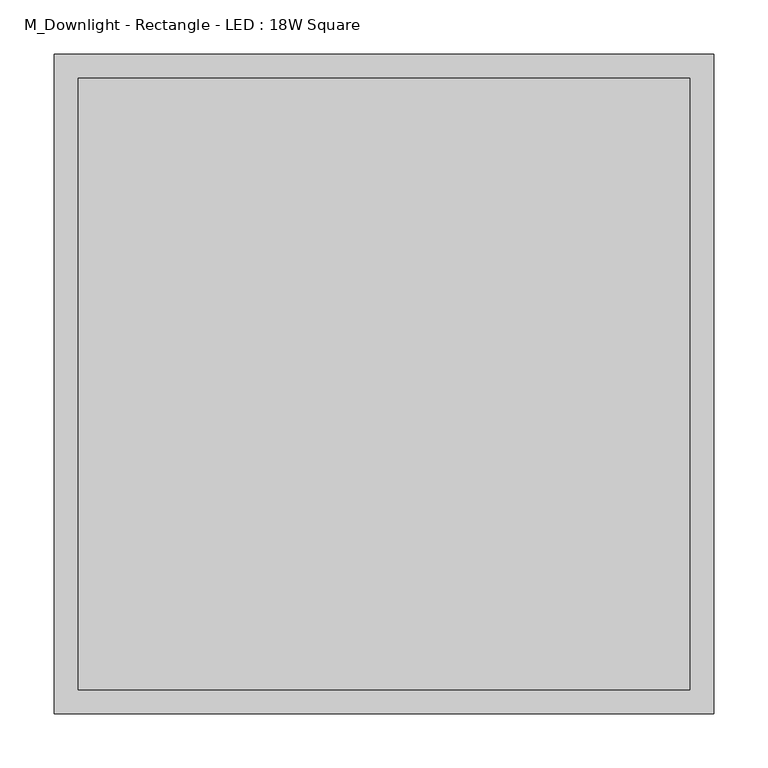
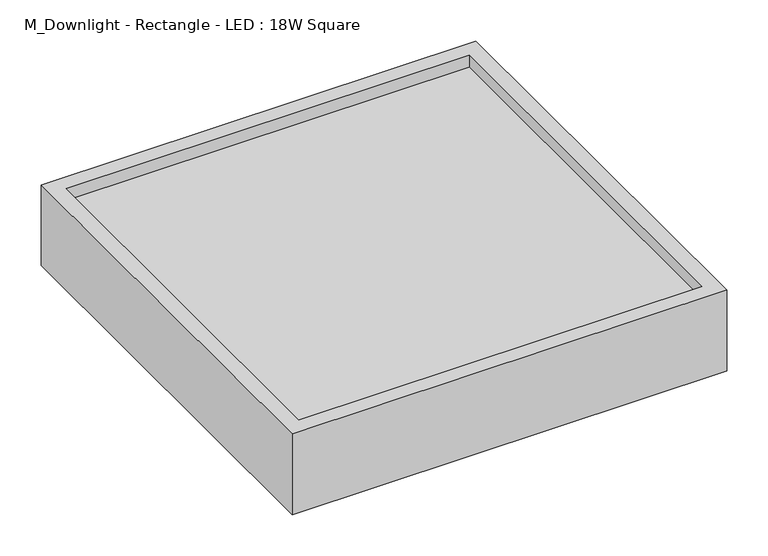
"""IFC4 building model written with IfcOpenShell, lengths in millimetres: light fixture geometry, M_Downlight - Rectangle - LED : 18W Square."""

from ifc_helpers import new_model, si_unit, frame, origin, place, context, project, spatial, polyline, outline, extrude, faceted_brep, source, transform, mapped, element, save


def m_downlight_rectangle_led_18w_square_4974df87(model_context):
    return source(origin(), model_context, "Body", "SolidModel", [
        extrude(outline(polyline([(282.775, 282.775), (282.775, -282.775), (-282.775, -282.775), (-282.775, 282.775), (282.775, 282.775)])), frame((0.0, 0.0, 84.7359902), z_axis=(0.0, 0.0, 1.0), x_axis=(1.0, 0.0, 0.0)), (0.0, 0.0, 1.0), 17.6320049),
        faceted_brep([(305.0, 305.0, 120.0), (-305.0, 305.0, 120.0), (-305.0, -305.0, 120.0), (305.0, -305.0, 120.0), (-282.775, 282.775, 120.0), (282.775, 282.775, 120.0), (282.775, -282.775, 120.0), (-282.775, -282.775, 120.0), (305.0, 305.0, 0.0), (305.0, -305.0, 0.0), (-305.0, -305.0, 0.0), (-305.0, 305.0, 0.0), (282.775, 282.775, 17.0719804), (-282.775, 282.775, 17.0719804), (-282.775, -282.775, 17.0719804), (282.775, -282.775, 17.0719804)], [[[0, 1, 2, 3], [4, 5, 6, 7]], [[8, 9, 10, 11]], [[1, 0, 8, 11]], [[2, 1, 11, 10]], [[3, 2, 10, 9]], [[0, 3, 9, 8]], [[12, 13, 14, 15]], [[13, 12, 5, 4]], [[14, 13, 4, 7]], [[15, 14, 7, 6]], [[12, 15, 6, 5]]]),
    ])


if __name__ == "__main__":
    model = new_model("IFC4")
    model_context = context("Model", 3, world=origin())
    ifc_project = project(units=[si_unit("LENGTHUNIT", "METRE", prefix="MILLI")], contexts=[model_context])
    site = spatial("IfcSite", under=ifc_project)
    building = spatial("IfcBuilding", under=site)
    placement = place(None, origin())
    m_downlight_rectangle_led_18w_square_shape = m_downlight_rectangle_led_18w_square_4974df87(model_context)
    element("IfcLightFixture", 1, ObjectType="M_Downlight - Rectangle - LED : 18W Square", at=placement, inside=building, context=model_context, shape_type="MappedRepresentation", body=[
        mapped(m_downlight_rectangle_led_18w_square_shape, transform((0.0, 0.0, 0.0), x_axis=(1.0, 0.0, 0.0), y_axis=(0.0, 1.0, 0.0), z_axis=(0.0, 0.0, 1.0))),
    ])
    save(model, "model.ifc")

# Revit data of these elements
# Type "M_Downlight - Rectangle - LED : 18W Square"
#   Photometric Web File = "2ACLX2_20L.ies"
#   Lamp = "LED"
#   Width = 0.61 m
#   Wattage = 18 W
#   built-in parameter 1150110 = 1 (stored number, unit not read)
#   Voltage = 120 V
#   built-in parameter 1114217 = 1 (stored number, unit not read)
#   Tilt Angle = 90.00°
#   built-in parameter 1150109 = 1 (stored number, unit not read)
#   built-in parameter 1150113 = 1 (stored number, unit not read)
#   built-in parameter 1150105 = 212.771 (stored number, unit not read)
#   Lumens = 2673.76 lm
#   built-in parameter 1150115 = 1 (stored number, unit not read)
#   Length = 0.61 m
#   built-in parameter 1150112 = 1 (stored number, unit not read)
#   built-in parameter 1150114 = 1 (stored number, unit not read)
#   built-in parameter 1150107 = 3200 (stored number, unit not read)
#   built-in parameter 1150106 = 2.12771 (stored number, unit not read)
#   Emit from Rectangle Width = 0.59095 m
#   Emit from Rectangle Length = 0.59095 m
#   built-in parameter 1150104 = 13.8 (stored number, unit not read)
#   Depth = 0.12 m
#   Default Elevation = 1.2 m
#   built-in parameter 1114218 = 1 (stored number, unit not read)
#   built-in parameter 1150133 = 10 (stored number, unit not read)
#   built-in parameter 1150134 = 3
#   Number of Poles = 1
#   Color Filter = 16777215
#   Load Classification = Lighting - Dwelling Unit
#   Shade Material = Metal - Paint Finish - Ivory, Glossy
#   Diffuser Material = Glass - White, High Luminance
#   Emit Shape Visible in Rendering = no
#   Dimming Lamp Color Temperature Shift = (empty or 0)
#   Apparent Load = 0
# Element 1 (IfcLightFixture, "M_Downlight - Rectangle - LED : 18W Square")
#   Materials on its faces: "Metal - Paint Finish - Ivory, Glossy", "Glass - White, High Luminance"
# Materials
#   "Metal - Paint Finish - Ivory, Glossy": class "Paint", colour RGB 247 247 239, transparency 0
#   "Glass - White, High Luminance": class "Glass", colour RGB 249 250 249, transparency 0.8
